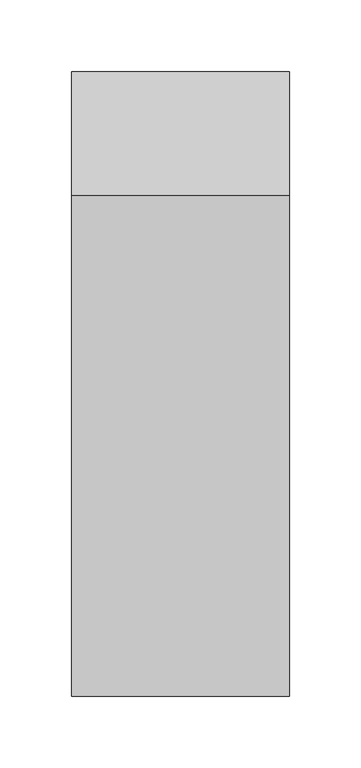
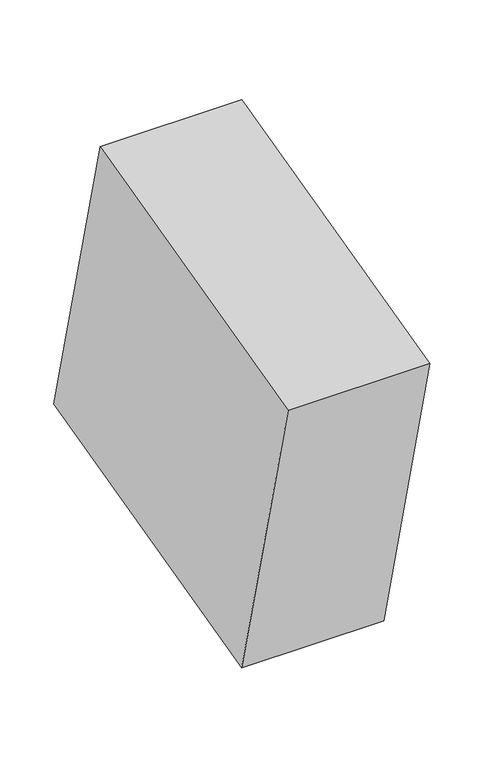
"""IFC4 building model written with IfcOpenShell, lengths in millimetres: proxy geometry, Framing018 3136 : Framing018 3136."""

from ifc_helpers import new_model, si_unit, frame, origin, place, context, project, spatial, polyline, outline, extrude, source, transform, mapped, element, save


def generic_models_7e24638c(model_context):
    return source(origin(), model_context, "Body", "SweptSolid", [
        extrude(outline(polyline([(10616.8128942, 43457.8953321), (10266.6377213, 43370.3515388), (10180.3882058, 43715.2646709), (10530.5446077, 43802.8723498), (10616.8128942, 43457.8953321)])), frame((5541.8883192, 0.0, 0.0), z_axis=(1.0, 0.0, 0.0), x_axis=(0.0, 1.0, 0.0)), (0.0, 0.0, 1.0), 152.4),
    ])


if __name__ == "__main__":
    model = new_model("IFC4")
    model_context = context("Model", 3, world=origin())
    ifc_project = project(units=[si_unit("LENGTHUNIT", "METRE", prefix="MILLI")], contexts=[model_context])
    site = spatial("IfcSite", under=ifc_project)
    building = spatial("IfcBuilding", under=site)
    placement = place(None, origin())
    generic_models_shape = generic_models_7e24638c(model_context)
    element("IfcBuildingElementProxy", 1, Name="Framing018 3136 : Framing018 3136", ObjectType="Framing018 3136 : Framing018 3136", at=placement, inside=building, context=model_context, shape_type="MappedRepresentation", body=[
        mapped(generic_models_shape, transform((0.0, 0.0, 0.0), x_axis=(1.0, 0.0, 0.0), y_axis=(0.0, 1.0, 0.0), z_axis=(0.0, 0.0, 1.0))),
    ])
    save(model, "model.ifc")

# Revit data of these elements
# Type "Framing018 3136 : Framing018 3136"
#   NameOverride = "Framing018"
# Element 1 (IfcBuildingElementProxy, "Framing018 3136 : Framing018 3136")
#   Materials on its faces: "WOOD FRAMING (SEE STRUCT DWGS)"
# Materials
#   "WOOD FRAMING (SEE STRUCT DWGS)": class "Unassigned", colour RGB 224 188 168, transparency 0, Cost = 0
